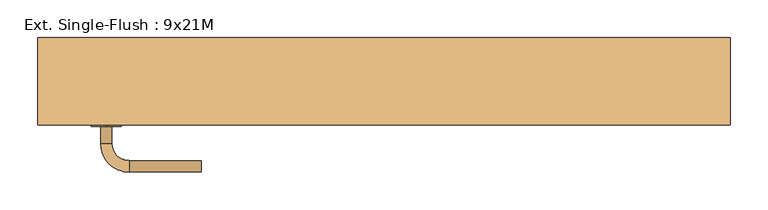
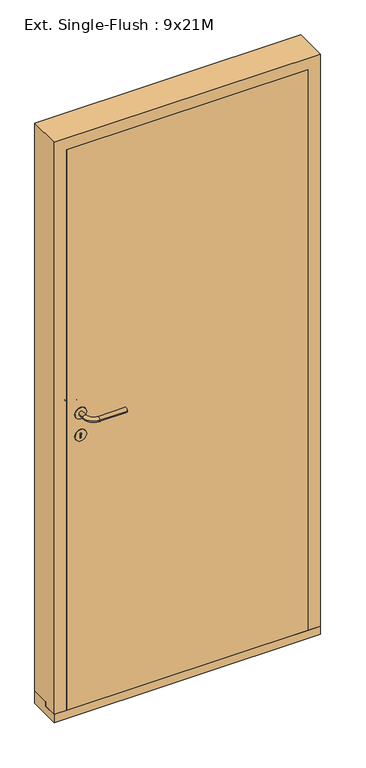
"""IFC4 building model written with IfcOpenShell, lengths in millimetres: door geometry, Ext. Single-Flush : 9x21M."""

from ifc_helpers import new_model, si_unit, point, frame, frame_2d, origin, place, context, project, spatial, polyline, circle_curve, ellipse_curve, trimmed, segment, composite_curve, outline, extrude, faceted_brep, source, transform, mapped, element, save
from ifc_brep_helpers import plane_surface, cylinder_surface, revolved_surface, advanced_brep


def ext_single_flush_9x21m_ea871c4f(model_context):
    return source(origin(), model_context, "Body", "SolidModel", [
        extrude(outline(composite_curve([segment(trimmed(circle_curve(frame_2d((1090.0, -366.0)), 20.0), [point((1070.0, -366.0))], [point((1110.0, -366.0))], False, "CARTESIAN"), True, "CONTINUOUS"), segment(trimmed(circle_curve(frame_2d((1090.0, -366.0)), 20.0), [point((1110.0, -366.0))], [point((1070.0, -366.0))], False, "CARTESIAN"), True, "CONTINUOUS")], self_intersect=False)), frame((0.0, -186.0, 0.0), z_axis=(0.0, 1.0, 0.0), x_axis=(0.0, 0.0, 1.0)), (0.0, 0.0, 1.0), 2.0),
        advanced_brep(
        [(-373.5, -186.0, 1090.0), (-358.5, -186.0, 1090.0), (-358.5, -208.5, 1090.0), (-373.5, -208.5, 1090.0), (-336.0, -231.0, 1090.0), (-336.0, -246.0, 1090.0), (-241.0, -231.0, 1090.0), (-241.0, -246.0, 1090.0)],
        [
            (0, 1, circle_curve(frame((-366.0, -186.0, 1090.0), z_axis=(0.0, 1.0, 0.0), x_axis=(1.0, 0.0, 0.0)), 7.5)),
            (1, 0, circle_curve(frame((-366.0, -186.0, 1090.0), z_axis=(0.0, 1.0, 0.0), x_axis=(1.0, 0.0, 0.0)), 7.5)),
            (1, 2),
            (2, 3, circle_curve(frame((-366.0, -208.5, 1090.0), z_axis=(0.0, 1.0, 0.0), x_axis=(1.0, 0.0, 0.0)), 7.5)),
            (3, 0),
            (3, 2, circle_curve(frame((-366.0, -208.5, 1090.0), z_axis=(0.0, 1.0, 0.0), x_axis=(1.0, 0.0, 0.0)), 7.5)),
            (4, 5, circle_curve(frame((-336.0, -238.5, 1090.0), z_axis=(-1.0, 0.0, 0.0), x_axis=(0.0, 1.0, 0.0)), 7.5)),
            (5, 3, circle_curve(frame((-336.0, -208.5, 1090.0), z_axis=(0.0, 0.0, -1.0), x_axis=(-1.0, 0.0, 0.0)), 37.5)),
            (2, 4, circle_curve(frame((-336.0, -208.5, 1090.0), z_axis=(0.0, 0.0, 1.0), x_axis=(-1.0, 0.0, 0.0)), 22.5)),
            (5, 4, circle_curve(frame((-336.0, -238.5, 1090.0), z_axis=(-1.0, 0.0, 0.0), x_axis=(0.0, 1.0, 0.0)), 7.5)),
            (4, 6),
            (6, 7, circle_curve(frame((-241.0, -238.5, 1090.0), z_axis=(-1.0, 0.0, 0.0), x_axis=(0.0, 1.0, 0.0)), 7.5)),
            (7, 5),
            (7, 6, circle_curve(frame((-241.0, -238.5, 1090.0), z_axis=(-1.0, 0.0, 0.0), x_axis=(0.0, 1.0, 0.0)), 7.5)),
        ],
        [
            plane_surface(frame((-366.0, -186.0, 1090.0), z_axis=(0.0, 1.0, 0.0), x_axis=(0.0, 0.0, -1.0))),
            cylinder_surface(frame((-366.0, -186.0, 1090.0), z_axis=(0.0, 1.0, 0.0), x_axis=(1.0, 0.0, 0.0)), 7.5),
            revolved_surface(trimmed(ellipse_curve(frame((-366.0, -208.5, 1090.0), z_axis=(0.0, -1.0, 0.0), x_axis=(1.0, 0.0, 0.0)), 7.5, 7.5), [point((-373.5, -208.5, 1090.0))], [point((-358.5, -208.5, 1090.0))], True, "CARTESIAN"), (-336.0, -208.5, 1090.0), (0.0, 0.0, -1.0)),
            revolved_surface(trimmed(ellipse_curve(frame((-366.0, -208.5, 1090.0), z_axis=(0.0, -1.0, 0.0), x_axis=(1.0, 0.0, 0.0)), 7.5, 7.5), [point((-358.5, -208.5, 1090.0))], [point((-373.5, -208.5, 1090.0))], True, "CARTESIAN"), (-336.0, -208.5, 1090.0), (0.0, 0.0, -1.0)),
            cylinder_surface(frame((-336.0, -238.5, 1090.0), z_axis=(-1.0, 0.0, 0.0), x_axis=(0.0, 1.0, 0.0)), 7.5),
            plane_surface(frame((-241.0, -238.5, 1090.0), z_axis=(1.0, 0.0, 0.0), x_axis=(0.0, 0.0, -1.0))),
        ],
        [
            (0, [[1, 2]]),
            (1, [[3, 4, 5, -2]]),
            (1, [[-5, 6, -3, -1]]),
            (2, [[7, 8, -4, 9]]),
            (3, [[10, -9, -6, -8]]),
            (4, [[11, 12, 13, -7]]),
            (4, [[-13, 14, -11, -10]]),
            (5, [[-12, -14]]),
        ],
    ),
        extrude(outline(composite_curve([segment(trimmed(circle_curve(frame_2d((1010.0, -366.0)), 20.0), [point((990.0, -366.0))], [point((1030.0, -366.0))], False, "CARTESIAN"), True, "CONTINUOUS"), segment(trimmed(circle_curve(frame_2d((1010.0, -366.0)), 20.0), [point((1030.0, -366.0))], [point((990.0, -366.0))], False, "CARTESIAN"), True, "CONTINUOUS")], self_intersect=False), holes=[composite_curve([segment(trimmed(circle_curve(frame_2d((1015.0, -366.0)), 3.0), [point((1012.4019238, -367.5))], [point((1012.4019238, -364.5))], True, "CARTESIAN"), True, "CONTINUOUS"), segment(polyline([(1012.4019238, -364.5), (1000.0, -364.5), (1000.0, -367.5), (1012.4019238, -367.5)]), True, "CONTINUOUS")], self_intersect=False)]), frame((0.0, -186.0, 0.0), z_axis=(0.0, 1.0, 0.0), x_axis=(0.0, 0.0, 1.0)), (0.0, 0.0, 1.0), 2.0),
        extrude(outline(composite_curve([segment(trimmed(circle_curve(frame_2d((1090.0, -366.0)), 20.0), [point((1070.0, -366.0))], [point((1110.0, -366.0))], False, "CARTESIAN"), True, "CONTINUOUS"), segment(trimmed(circle_curve(frame_2d((1090.0, -366.0)), 20.0), [point((1110.0, -366.0))], [point((1070.0, -366.0))], False, "CARTESIAN"), True, "CONTINUOUS")], self_intersect=False)), frame((0.0, -134.0, 0.0), z_axis=(0.0, 1.0, 0.0), x_axis=(0.0, 0.0, 1.0)), (0.0, 0.0, 1.0), 2.0),
        advanced_brep(
        [(-373.5, -132.0, 1090.0), (-358.5, -132.0, 1090.0), (-373.5, -109.5, 1090.0), (-358.5, -109.5, 1090.0), (-336.0, -87.0, 1090.0), (-336.0, -72.0, 1090.0), (-241.0, -72.0, 1090.0), (-241.0, -87.0, 1090.0)],
        [
            (0, 1, circle_curve(frame((-366.0, -132.0, 1090.0), z_axis=(0.0, -1.0, 0.0), x_axis=(1.0, 0.0, 0.0)), 7.5)),
            (1, 0, circle_curve(frame((-366.0, -132.0, 1090.0), z_axis=(0.0, -1.0, 0.0), x_axis=(1.0, 0.0, 0.0)), 7.5)),
            (0, 2),
            (2, 3, circle_curve(frame((-366.0, -109.5, 1090.0), z_axis=(0.0, -1.0, 0.0), x_axis=(1.0, 0.0, 0.0)), 7.5)),
            (3, 1),
            (3, 2, circle_curve(frame((-366.0, -109.5, 1090.0), z_axis=(0.0, -1.0, 0.0), x_axis=(1.0, 0.0, 0.0)), 7.5)),
            (4, 3, circle_curve(frame((-336.0, -109.5, 1090.0), z_axis=(0.0, 0.0, 1.0), x_axis=(-1.0, 0.0, 0.0)), 22.5)),
            (2, 5, circle_curve(frame((-336.0, -109.5, 1090.0), z_axis=(0.0, 0.0, -1.0), x_axis=(-1.0, 0.0, 0.0)), 37.5)),
            (5, 4, circle_curve(frame((-336.0, -79.5, 1090.0), z_axis=(-1.0, 0.0, 0.0), x_axis=(0.0, -1.0, 0.0)), 7.5)),
            (4, 5, circle_curve(frame((-336.0, -79.5, 1090.0), z_axis=(-1.0, 0.0, 0.0), x_axis=(0.0, -1.0, 0.0)), 7.5)),
            (5, 6),
            (6, 7, circle_curve(frame((-241.0, -79.5, 1090.0), z_axis=(-1.0, 0.0, 0.0), x_axis=(0.0, -1.0, 0.0)), 7.5)),
            (7, 4),
            (7, 6, circle_curve(frame((-241.0, -79.5, 1090.0), z_axis=(-1.0, 0.0, 0.0), x_axis=(0.0, -1.0, 0.0)), 7.5)),
        ],
        [
            plane_surface(frame((-366.0, -132.0, 1090.0), z_axis=(0.0, -1.0, 0.0), x_axis=(0.0, 0.0, -1.0))),
            cylinder_surface(frame((-366.0, -132.0, 1090.0), z_axis=(0.0, -1.0, 0.0), x_axis=(1.0, 0.0, 0.0)), 7.5),
            revolved_surface(trimmed(ellipse_curve(frame((-366.0, -109.5, 1090.0), z_axis=(0.0, -1.0, 0.0), x_axis=(1.0, 0.0, 0.0)), 7.5, 7.5), [point((-373.5, -109.5, 1090.0))], [point((-358.5, -109.5, 1090.0))], True, "CARTESIAN"), (-336.0, -109.5, 1090.0), (0.0, 0.0, -1.0)),
            revolved_surface(trimmed(ellipse_curve(frame((-366.0, -109.5, 1090.0), z_axis=(0.0, -1.0, 0.0), x_axis=(1.0, 0.0, 0.0)), 7.5, 7.5), [point((-358.5, -109.5, 1090.0))], [point((-373.5, -109.5, 1090.0))], True, "CARTESIAN"), (-336.0, -109.5, 1090.0), (0.0, 0.0, -1.0)),
            cylinder_surface(frame((-336.0, -79.5, 1090.0), z_axis=(-1.0, 0.0, 0.0), x_axis=(0.0, -1.0, 0.0)), 7.5),
            plane_surface(frame((-241.0, -79.5, 1090.0), z_axis=(1.0, 0.0, 0.0), x_axis=(0.0, 0.0, -1.0))),
        ],
        [
            (0, [[1, 2]]),
            (1, [[-1, 3, 4, 5]]),
            (1, [[-2, -5, 6, -3]]),
            (2, [[7, -4, 8, 9]]),
            (3, [[-8, -6, -7, 10]]),
            (4, [[-9, 11, 12, 13]]),
            (4, [[-10, -13, 14, -11]]),
            (5, [[-14, -12]]),
        ],
    ),
        extrude(outline(composite_curve([segment(trimmed(circle_curve(frame_2d((1010.0, -366.0)), 20.0), [point((990.0, -366.0))], [point((1030.0, -366.0))], False, "CARTESIAN"), True, "CONTINUOUS"), segment(trimmed(circle_curve(frame_2d((1010.0, -366.0)), 20.0), [point((1030.0, -366.0))], [point((990.0, -366.0))], False, "CARTESIAN"), True, "CONTINUOUS")], self_intersect=False), holes=[composite_curve([segment(trimmed(circle_curve(frame_2d((1015.0, -366.0)), 3.0), [point((1012.4019238, -367.5))], [point((1012.4019238, -364.5))], True, "CARTESIAN"), True, "CONTINUOUS"), segment(polyline([(1012.4019238, -364.5), (1000.0, -364.5), (1000.0, -367.5), (1012.4019238, -367.5)]), True, "CONTINUOUS")], self_intersect=False)]), frame((0.0, -134.0, 0.0), z_axis=(0.0, 1.0, 0.0), x_axis=(0.0, 0.0, 1.0)), (0.0, 0.0, 1.0), 2.0),
        extrude(outline(polyline([(-414.0, -184.0), (-414.0, -134.0), (414.0, -134.0), (414.0, -184.0), (-414.0, -184.0)])), frame((0.0, 0.0, 30.0), z_axis=(0.0, 0.0, 1.0), x_axis=(1.0, 0.0, 0.0)), (0.0, 0.0, 1.0), 2028.0),
        faceted_brep([(414.0, -184.0, 2058.0), (414.0, -184.0, 30.0), (456.0, -184.0, 30.0), (456.0, -184.0, 2100.0), (-456.0, -184.0, 2100.0), (-456.0, -184.0, 30.0), (-414.0, -184.0, 30.0), (-414.0, -184.0, 2058.0), (-414.0, -134.0, 30.0), (-414.0, -134.0, 45.0), (-414.0, -134.0, 2058.0), (-456.0, -134.0, 30.0), (456.0, -134.0, 30.0), (414.0, -134.0, 30.0), (-456.0, -69.0, 2100.0), (-456.0, -69.0, 45.0), (-456.0, -134.0, 45.0), (456.0, -134.0, 45.0), (456.0, -69.0, 45.0), (456.0, -69.0, 2100.0), (414.0, -134.0, 2058.0), (414.0, -134.0, 45.0), (399.0, -69.0, 45.0), (399.0, -69.0, 2043.0), (-399.0, -69.0, 2043.0), (-399.0, -69.0, 45.0), (-399.0, -134.0, 45.0), (399.0, -134.0, 45.0), (-399.0, -134.0, 2043.0), (399.0, -134.0, 2043.0)], [[[0, 1, 2, 3, 4, 5, 6, 7]], [[7, 6, 8, 9, 10]], [[8, 6, 5, 11]], [[12, 2, 1, 13]], [[14, 15, 16, 11, 5, 4]], [[3, 2, 12, 17, 18, 19]], [[20, 21, 13, 1, 0]], [[19, 18, 22, 23, 24, 25, 15, 14]], [[16, 15, 25, 26, 9]], [[21, 27, 22, 18, 17]], [[9, 8, 11, 16]], [[17, 12, 13, 21]], [[28, 26, 25, 24]], [[23, 22, 27, 29]], [[29, 27, 21, 20, 10, 9, 26, 28]], [[3, 19, 14, 4]], [[23, 29, 28, 24]], [[7, 10, 20, 0]]]),
        extrude(outline(polyline([(-184.0, 30.0), (-134.0, 30.0), (-134.0, 45.0), (-69.0, 45.0), (-69.0, 0.0), (-184.0, 0.0), (-184.0, 30.0)])), frame((-456.0, 0.0, 0.0), z_axis=(1.0, 0.0, 0.0), x_axis=(0.0, 1.0, 0.0)), (0.0, 0.0, 1.0), 912.0),
    ])


if __name__ == "__main__":
    model = new_model("IFC4")
    model_context = context("Model", 3, world=origin())
    ifc_project = project(units=[si_unit("LENGTHUNIT", "METRE", prefix="MILLI")], contexts=[model_context])
    site = spatial("IfcSite", under=ifc_project)
    building = spatial("IfcBuilding", under=site)
    placement = place(None, origin())
    ext_single_flush_9x21m_shape = ext_single_flush_9x21m_ea871c4f(model_context)
    element("IfcDoor", 1, ObjectType="Ext. Single-Flush : 9x21M", at=placement, inside=building, context=model_context, shape_type="MappedRepresentation", body=[
        mapped(ext_single_flush_9x21m_shape, transform((0.0, 0.0, 0.0), x_axis=(1.0, 0.0, 0.0), y_axis=(0.0, 1.0, 0.0), z_axis=(0.0, 0.0, 1.0))),
    ])
    save(model, "model.ifc")

# Revit data of these elements
# Type "Ext. Single-Flush : 9x21M"
#   Type Mark = "51"
#   Sound Rating = ""
#   Opening Side [instance default] = ""
#   Hinge Side [instance default] = ""
#   Creator Organization [instance default] = "© Danish Educational Content"
#   Creator Name [instance default] = "© Erik Falck Jørgensen"
#   Creator Build [instance default] = "2017.0301.0"
#   Analytic Construction = "<None>"
#   length#6 = -50 mm
#   length#5 = 912 mm
#   length#4 = 120 mm
#   length#3 = 30 mm
#   length#2 = 57 mm
#   length#1 = 0 mm
#   Thickness = 50 mm
#   Seal Width = 12 mm
#   Rough Width = 912 mm
#   Rough Height = 2100 mm
#   Rebate Depth = 50 mm
#   Rabbet Width = 15 mm
#   Rabbet Depth = 50 mm
#   Height = 2088 mm
#   Width = 888 mm
#   Handle From Side = 90 mm
#   Handle From Bottom = 1090 mm
#   Exterior Direction [instance default] = 0.00°
#   Case Width = 45 mm
#   Case Depth = 115 mm
#   Threshold = yes
#   Sealing = no
#   Hinging = yes
#   Wall Closure = 1
#   Function = 1
#   Panel = none
#   Handle Finish = none
#   Handle = element 507533
#   Embrasure Interior = none
#   Embrasure Exterior = none
#   Case/Transom = none
#   Assembly Code = ""
# Element 1 (IfcDoor, "Ext. Single-Flush : 9x21M")
#   Materials on its faces: "Stainless Steel, Polished", "Default Frame/Mullion (Interior/Exterior)", "Default Door Panel (Exterior/Interior)"
# Materials
#   "Stainless Steel, Polished": class "Metal", colour RGB 180 180 180, transparency 0, Description = "Rustfri stål, poleret", Cost = 0
#   "Default Frame/Mullion (Interior/Exterior)": class "Generic", colour RGB 205 205 205, transparency 0, Description = "Udefineret karm/ramme materiale", Cost = 0
#   "Default Door Panel (Exterior/Interior)": class "Generic", colour RGB 205 205 205, transparency 0, Description = "Udefineret dørplade materiale", Cost = 0
